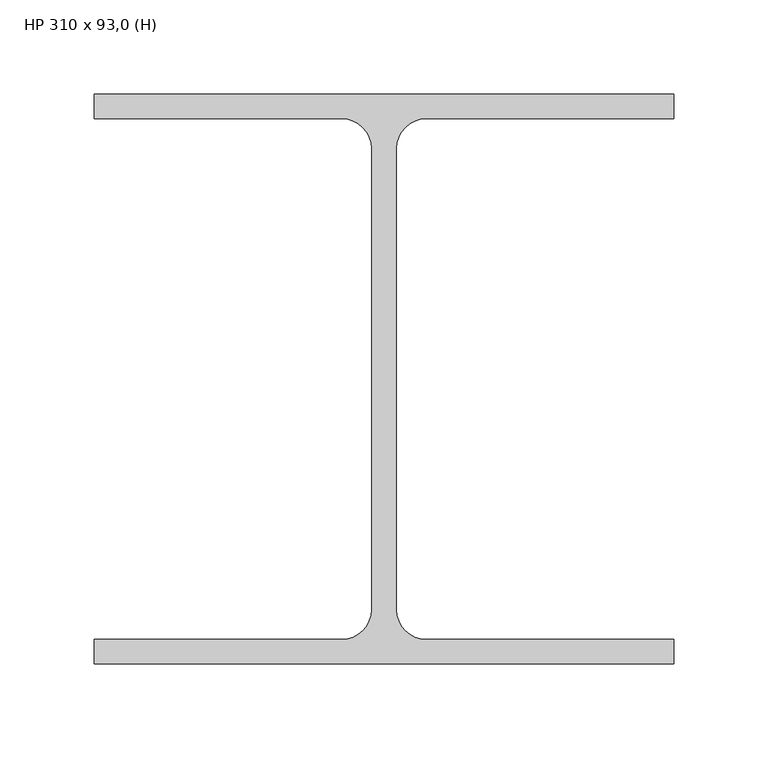
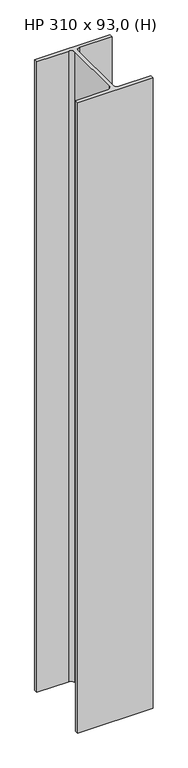
"""IFC4 building model written with IfcOpenShell, lengths in millimetres: column geometry, Pilar de Aço - H : HP 310 x 93,0 (H)."""

from ifc_helpers import new_model, si_unit, point, frame_2d, origin, origin_with_axes, place, context, project, spatial, polyline, circle_curve, trimmed, segment, composite_curve, outline, extrude, source, transform, mapped, element, save


def hp_310_x_93_0_h_2d520116(model_context):
    return source(origin(), model_context, "Body", "SweptSolid", [
        extrude(outline(composite_curve([segment(polyline([(154.0, 151.5), (154.0, 138.4), (22.45, 138.4)]), True, "CONTINUOUS"), segment(trimmed(circle_curve(frame_2d((22.45, 122.5)), 15.9), [point((22.45, 138.4))], [point((6.55, 122.5))], True, "CARTESIAN"), True, "CONTINUOUS"), segment(polyline([(6.55, 122.5), (6.55, -122.5)]), True, "CONTINUOUS"), segment(trimmed(circle_curve(frame_2d((22.45, -122.5)), 15.9), [point((6.55, -122.5))], [point((22.45, -138.4))], True, "CARTESIAN"), True, "CONTINUOUS"), segment(polyline([(22.45, -138.4), (154.0, -138.4), (154.0, -151.5), (-154.0, -151.5), (-154.0, -138.4), (-22.45, -138.4)]), True, "CONTINUOUS"), segment(trimmed(circle_curve(frame_2d((-22.45, -122.5)), 15.9), [point((-22.45, -138.4))], [point((-6.55, -122.5))], True, "CARTESIAN"), True, "CONTINUOUS"), segment(polyline([(-6.55, -122.5), (-6.55, 122.5)]), True, "CONTINUOUS"), segment(trimmed(circle_curve(frame_2d((-22.45, 122.5)), 15.9), [point((-6.55, 122.5))], [point((-22.45, 138.4))], True, "CARTESIAN"), True, "CONTINUOUS"), segment(polyline([(-22.45, 138.4), (-154.0, 138.4), (-154.0, 151.5), (154.0, 151.5)]), True, "CONTINUOUS")], self_intersect=False)), origin_with_axes(), (0.0, 0.0, 1.0), 2720.0),
    ])


if __name__ == "__main__":
    model = new_model("IFC4")
    model_context = context("Model", 3, world=origin())
    ifc_project = project(units=[si_unit("LENGTHUNIT", "METRE", prefix="MILLI")], contexts=[model_context])
    site = spatial("IfcSite", under=ifc_project)
    building = spatial("IfcBuilding", under=site)
    placement = place(None, origin())
    hp_310_x_93_0_h_shape = hp_310_x_93_0_h_2d520116(model_context)
    element("IfcColumn", 1, ObjectType="Pilar de Aço - H : HP 310 x 93,0 (H)", at=placement, inside=building, context=model_context, shape_type="MappedRepresentation", body=[
        mapped(hp_310_x_93_0_h_shape, transform((0.0, 0.0, 0.0), x_axis=(1.0, 0.0, 0.0), y_axis=(0.0, 1.0, 0.0), z_axis=(0.0, 0.0, 1.0))),
    ])
    save(model, "model.ifc")

# Revit data of these elements
# Type "Pilar de Aço - H : HP 310 x 93,0 (H)"
#   SINAPI = ""
#   Área da seção = 119.2 m²
#   tw = 1.31 cm
#   tf = 1.31 cm
#   h = 27.68 cm
#   d' = 24.50 cm
#   d = 30.30 cm
#   bf = 30.80 cm
#   R = 1.59 cm
#   Massa Linear kg/m = 93
#   Aço = Metal - Aço 345MPa
#   Assembly Code = ""
# Materials
#   "Metal - Aço 345MPa": class "Metal", colour RGB 189 187 185, transparency 0, Cost = 0
